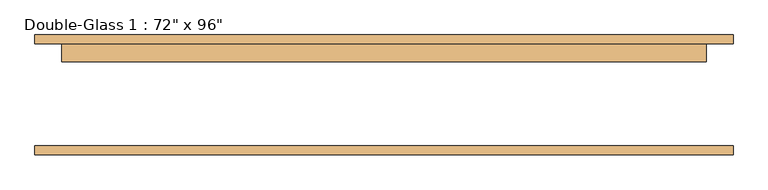
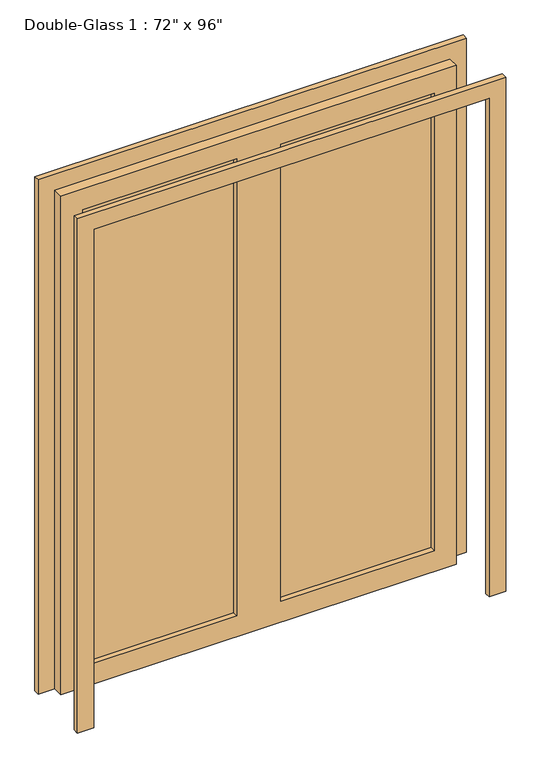
"""IFC4 building model written with IfcOpenShell, lengths in millimetres: door geometry."""

from ifc_helpers import new_model, si_unit, frame, origin, place, context, project, spatial, polyline, outline, extrude, source, transform, mapped, element, save


def door_b879888b(model_context):
    return source(origin(), model_context, "Body", "SweptSolid", [
        extrude(outline(polyline([(0.0, 990.6), (2514.6, 990.6), (2514.6, -990.6), (0.0, -990.6), (0.0, -914.4), (2438.4, -914.4), (2438.4, 914.4), (0.0, 914.4), (0.0, 990.6)])), frame((0.0, -167.48125, 0.0), z_axis=(0.0, 1.0, 0.0), x_axis=(0.0, 0.0, 1.0)), (0.0, 0.0, 1.0), 25.4),
        extrude(outline(polyline([(2438.4, 914.4), (0.0, 914.4), (0.0, 990.6), (2514.6, 990.6), (2514.6, -990.6), (0.0, -990.6), (0.0, -914.4), (2438.4, -914.4), (2438.4, 914.4)])), frame((0.0, 146.84375, 0.0), z_axis=(0.0, 1.0, 0.0), x_axis=(0.0, 0.0, 1.0)), (0.0, 0.0, 1.0), 25.4),
        extrude(outline(polyline([(812.8, 121.44375), (101.6, 121.44375), (101.6, 128.5875), (812.8, 128.5875), (812.8, 121.44375)])), frame((0.0, 0.0, 101.6), z_axis=(0.0, 0.0, 1.0), x_axis=(1.0, 0.0, 0.0)), (0.0, 0.0, 1.0), 2235.2),
        extrude(outline(polyline([(-101.6, 121.44375), (-812.8, 121.44375), (-812.8, 128.5875), (-101.6, 128.5875), (-101.6, 121.44375)])), frame((0.0, 0.0, 101.6), z_axis=(0.0, 0.0, 1.0), x_axis=(1.0, 0.0, 0.0)), (0.0, 0.0, 1.0), 2235.2),
        extrude(outline(polyline([(2438.4, 914.4), (2438.4, -914.4), (0.0, -914.4), (0.0, 914.4), (2438.4, 914.4)]), holes=[polyline([(2336.8, -101.6), (101.6, -101.6), (101.6, -812.8), (2336.8, -812.8), (2336.8, -101.6)]), polyline([(2336.8, 812.8), (101.6, 812.8), (101.6, 101.6), (2336.8, 101.6), (2336.8, 812.8)])]), frame((0.0, 96.04375, 0.0), z_axis=(0.0, 1.0, 0.0), x_axis=(0.0, 0.0, 1.0)), (0.0, 0.0, 1.0), 50.8),
    ])


if __name__ == "__main__":
    model = new_model("IFC4")
    model_context = context("Model", 3, world=origin())
    ifc_project = project(units=[si_unit("LENGTHUNIT", "METRE", prefix="MILLI")], contexts=[model_context])
    site = spatial("IfcSite", under=ifc_project)
    building = spatial("IfcBuilding", under=site)
    placement = place(None, origin())
    door_shape = door_b879888b(model_context)
    element("IfcDoor", 1, ObjectType="Double-Glass 1 : 72\" x 96\"", at=placement, inside=building, context=model_context, shape_type="MappedRepresentation", body=[
        mapped(door_shape, transform((0.0, 0.0, 0.0), x_axis=(1.0, 0.0, 0.0), y_axis=(0.0, 1.0, 0.0), z_axis=(0.0, 0.0, 1.0))),
    ])
    save(model, "model.ifc")

# Revit data of these elements
# Type "Double-Glass 1 : 72\" x 96\""
#   Type Mark = "30"
#   Construction Type Id = "MDOOR"
#   Assembly Code = "C1020"
#   Analytic Construction = "Metal"
#   Thickness = 0' - 2"
#   Thermal Resistance (R) = 0.270118 (m²·K)/W
#   Heat Transfer Coefficient (U) = 3.70223 W/(m²·K)
#   Height = 8' - 0"
#   Rail Width - Base = 0' - 4"
#   Rail Width - Top = 0' - 4"
#   Stile Width - Hinge = 0' - 4"
#   Stile Width - Latch = 0' - 4"
#   Trim Projection = 0' - 1"
#   Trim Width = 0' - 3"
#   Width = 6' - 0"
#   Door Material = Aluminum
#   Frame Material = Aluminum
#   Visual Light Transmittance = 0
#   Solar Heat Gain Coefficient = 0
#   Function = (empty or 0)
#   Wall Closure = (empty or 0)
# Element 1 (IfcDoor, "Double-Glass 1 : 72\" x 96\"")
#   Materials on its faces: "Aluminum", "Glass"
# Materials
#   "Aluminum": class "Metal", colour RGB 226 226 226, transparency 0, Description = "Aluminum 6061", Cost = 0
#   "Glass": class "Glass", colour RGB 142 168 196, transparency 0.75, Description = "Soda Lime Glass", Cost = 0
